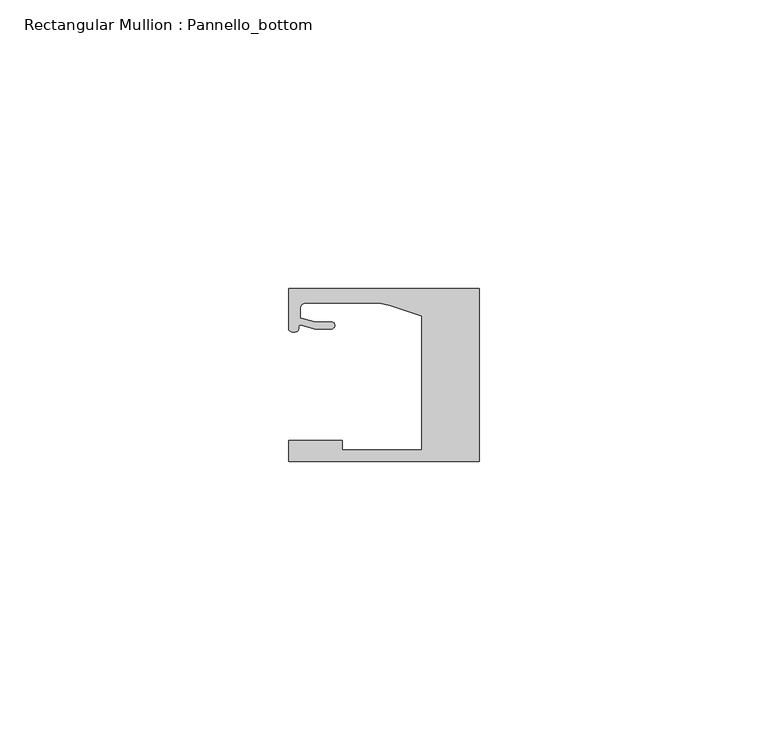
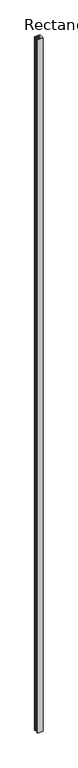
"""IFC4 building model written with IfcOpenShell, lengths in millimetres: member geometry, Rectangular Mullion : Pannello_bottom."""

import ifcopenshell
import ifcopenshell.guid

model = None  # the IFC model being written
_history = None  # IfcOwnerHistory: only IFC2X3 demands one
_inside = {}  # id of a spatial element -> (the spatial element, [elements in it])
_under = {}  # id of a project, library or spatial element -> (it, [spatial elements below it])
_declared = {}  # id of a project -> (the project, [libraries it declares])
_typed = {}  # id of a type object -> (the type object, [elements of that type])
_made_of = {}  # id of a material, layer set ... -> (it, [elements and type objects made of it])


def new_model(schema):
    """Start an empty IFC model of exactly this schema.

    Asked for "IFC4X3", IfcOpenShell would pick the latest addendum, in which some entities
    have other attributes; the version numbers below select the first issue.
    IFC2X3 requires an IfcOwnerHistory on every rooted entity: one is made here for all.
    """
    global model, _history
    if schema == "IFC4X3":
        model = ifcopenshell.file(schema_version=(4, 3, 0, 0))
    else:
        model = ifcopenshell.file(schema=schema)
    _inside.clear()
    _under.clear()
    _declared.clear()
    _typed.clear()
    _made_of.clear()
    _history = None
    if model.schema == "IFC2X3":
        org = make("IfcOrganization", Name="unknown")
        user = make(
            "IfcPersonAndOrganization",
            ThePerson=make("IfcPerson", FamilyName="unknown"),
            TheOrganization=org,
        )
        app = make(
            "IfcApplication",
            ApplicationDeveloper=org,
            Version="unknown",
            ApplicationFullName="unknown",
            ApplicationIdentifier="unknown",
        )
        _history = make(
            "IfcOwnerHistory",
            OwningUser=user,
            OwningApplication=app,
            ChangeAction="ADDED",
            CreationDate=0,
        )
    return model


def make(cls, **values):
    """One entity of the class cls with the attributes given. An attribute that is None is left unset."""
    return model.create_entity(
        cls, **{name: value for name, value in values.items() if value is not None}
    )


def rooted(cls, **values):
    """An entity with a GlobalId (a new one), such as an element, a storey or a relation."""
    return make(cls, GlobalId=ifcopenshell.guid.new(), OwnerHistory=_history, **values)


def si_unit(unit_type, name, prefix=None):
    """IfcSIUnit, for example si_unit("LENGTHUNIT", "METRE", prefix="MILLI")."""
    return make("IfcSIUnit", UnitType=unit_type, Prefix=prefix, Name=name)


def assignment(units):
    """IfcUnitAssignment: the units of a project."""
    return None if units is None else make("IfcUnitAssignment", Units=units)


def point(xyz):
    """IfcCartesianPoint."""
    return None if xyz is None else make("IfcCartesianPoint", Coordinates=xyz)


def direction(xyz):
    """IfcDirection."""
    return None if xyz is None else make("IfcDirection", DirectionRatios=xyz)


def frame(location, z_axis=None, x_axis=None):
    """IfcAxis2Placement3D, a coordinate frame: its origin and axes. An axis left out is left unset."""
    return make(
        "IfcAxis2Placement3D",
        Location=point(location),
        Axis=direction(z_axis),
        RefDirection=direction(x_axis),
    )


def origin():
    """The frame at (0, 0, 0) with its axes left unset."""
    return frame((0.0, 0.0, 0.0))


def place(relative_to, where):
    """IfcLocalPlacement: puts the frame where relative to a parent placement (None: the world)."""
    return make(
        "IfcLocalPlacement", PlacementRelTo=relative_to, RelativePlacement=where
    )


def context(
    kind, dimensions, precision=None, world=None, true_north=None, identifier=None
):
    """IfcGeometricRepresentationContext, for example the 3D "Model" context."""
    return make(
        "IfcGeometricRepresentationContext",
        ContextIdentifier=identifier,
        ContextType=kind,
        CoordinateSpaceDimension=dimensions,
        Precision=precision,
        WorldCoordinateSystem=world,
        TrueNorth=true_north,
    )


def project(units=None, contexts=None):
    """IfcProject with its units and contexts."""
    return rooted(
        "IfcProject",
        Name="project",
        RepresentationContexts=contexts,
        UnitsInContext=assignment(units),
    )


def spatial(cls, under=None, at=None, **own):
    """A site, building, storey or space (cls), placed at a placement, below another one or the project."""
    s = rooted(cls, ObjectPlacement=at, **own)
    if under is not None:
        _under.setdefault(under.id(), (under, []))[1].append(s)
    return s


def polyline(points):
    """IfcPolyline through the points."""
    return make("IfcPolyline", Points=[point(p) for p in points])


def circle_curve(where, radius):
    """IfcCircle in the frame where."""
    return make("IfcCircle", Position=where, Radius=radius)


def shape(context_of_items, identifier, shape_type, items):
    """IfcShapeRepresentation: the items that make up one representation, for example the "Body"."""
    return make(
        "IfcShapeRepresentation",
        ContextOfItems=context_of_items,
        RepresentationIdentifier=identifier,
        RepresentationType=shape_type,
        Items=items,
    )


def source(mapping_origin, context_of_items, identifier, shape_type, items):
    """IfcRepresentationMap: a shape defined once, which mapped items show again and again."""
    return make(
        "IfcRepresentationMap",
        MappingOrigin=mapping_origin,
        MappedRepresentation=shape(context_of_items, identifier, shape_type, items),
    )


def transform(
    local_origin,
    x_axis=None,
    y_axis=None,
    z_axis=None,
    scale=None,
    scale2=None,
    scale3=None,
    uniform=True,
):
    """IfcCartesianTransformationOperator3D, or its non-uniform kind. x_axis, y_axis, z_axis: its Axis1, 2, 3."""
    if uniform:
        return make(
            "IfcCartesianTransformationOperator3D",
            Axis1=direction(x_axis),
            Axis2=direction(y_axis),
            LocalOrigin=point(local_origin),
            Scale=scale,
            Axis3=direction(z_axis),
        )
    return make(
        "IfcCartesianTransformationOperator3DnonUniform",
        Axis1=direction(x_axis),
        Axis2=direction(y_axis),
        LocalOrigin=point(local_origin),
        Scale=scale,
        Axis3=direction(z_axis),
        Scale2=scale2,
        Scale3=scale3,
    )


def mapped(mapping_source, mapping_target):
    """IfcMappedItem: shows the shape of a source again, moved by a transform."""
    return make(
        "IfcMappedItem", MappingSource=mapping_source, MappingTarget=mapping_target
    )


def made_of(thing, what):
    """Note that an element or type object is made of a material, layer set ...; save() writes the relation."""
    if what is not None:
        _made_of.setdefault(what.id(), (what, []))[1].append(thing)
    return thing


def element(
    cls,
    number,
    at=None,
    inside=None,
    cuts=None,
    type_object=None,
    material=None,
    context=None,
    identifier="Body",
    shape_type=None,
    held_by="IfcProductDefinitionShape",
    body=None,
    shapes=None,
    **own,
):
    """One element of the class cls, such as IfcWall. Its Tag is "e" and its number.

    at: its placement. inside: the storey or other place that contains it. cuts: it is an
    opening in that element (IfcRelVoidsElement). A single representation is given by context,
    identifier, shape_type and body (its items); several are given by shapes. held_by: the class
    of the entity that holds the representations. save() writes the other relations.
    """
    e = rooted(cls, Tag="e%d" % number, ObjectPlacement=at, **own)
    if body is not None:
        shapes = [shape(context, identifier, shape_type, body)]
    if shapes is not None:
        e.Representation = make(held_by, Representations=shapes)
    if inside is not None:
        _inside.setdefault(inside.id(), (inside, []))[1].append(e)
    if cuts is not None:
        rooted(
            "IfcRelVoidsElement", RelatingBuildingElement=cuts, RelatedOpeningElement=e
        )
    if type_object is not None:
        _typed.setdefault(type_object.id(), (type_object, []))[1].append(e)
    return made_of(e, material)


def aggregate(whole, parts):
    """IfcRelAggregates: a whole, such as a stair, and the parts it consists of."""
    return rooted("IfcRelAggregates", RelatingObject=whole, RelatedObjects=parts)


def save(model, path):
    """Write the relations noted so far, then the file.

    IfcRelAggregates (storeys below a building ...), IfcRelContainedInSpatialStructure (elements
    in a storey), IfcRelDefinesByType, IfcRelAssociatesMaterial and IfcRelDeclares: one each for
    every whole, place, type object, material and project.
    """
    for whole, parts in _under.values():
        aggregate(whole, parts)
    for where, things in _inside.values():
        rooted(
            "IfcRelContainedInSpatialStructure",
            RelatedElements=things,
            RelatingStructure=where,
        )
    for kind, things in _typed.values():
        rooted("IfcRelDefinesByType", RelatedObjects=things, RelatingType=kind)
    for what, things in _made_of.values():
        rooted("IfcRelAssociatesMaterial", RelatedObjects=things, RelatingMaterial=what)
    for by, libraries in _declared.values():
        rooted("IfcRelDeclares", RelatingContext=by, RelatedDefinitions=libraries)
    model.write(path)


def plane_surface(at):
    """IfcPlane: the flat surface through the origin of the frame at, square to its z axis."""
    return make("IfcPlane", Position=at)


def cylinder_surface(at, radius):
    """IfcCylindricalSurface: all points at the distance radius from the z axis of the frame at."""
    return make("IfcCylindricalSurface", Position=at, Radius=radius)


def revolved_surface(curve, axis_point, axis_direction):
    """IfcSurfaceOfRevolution: the curve turned about the line through axis_point along axis_direction."""
    return make(
        "IfcSurfaceOfRevolution",
        SweptCurve=make("IfcArbitraryOpenProfileDef", ProfileType="CURVE", Curve=curve),
        AxisPosition=make("IfcAxis1Placement", Location=point(axis_point), Axis=direction(axis_direction)),
    )


def extruded_surface(curve, direction_of_extrusion, depth):
    """IfcSurfaceOfLinearExtrusion: the curve pushed along a direction by depth."""
    return make(
        "IfcSurfaceOfLinearExtrusion",
        SweptCurve=make("IfcArbitraryOpenProfileDef", ProfileType="CURVE", Curve=curve),
        ExtrudedDirection=direction(direction_of_extrusion),
        Depth=depth,
    )


def spline_curve(degree, points, multiplicities, knots, weights=None):
    """IfcBSplineCurveWithKnots; with weights, IfcRationalBSplineCurveWithKnots."""
    own = dict(
        Degree=degree,
        ControlPointsList=[point(p) for p in points],
        CurveForm="UNSPECIFIED",
        ClosedCurve=False,
        SelfIntersect=False,
        KnotMultiplicities=multiplicities,
        Knots=knots,
        KnotSpec="UNSPECIFIED",
    )
    if weights is None:
        return make("IfcBSplineCurveWithKnots", **own)
    return make("IfcRationalBSplineCurveWithKnots", WeightsData=weights, **own)


def advanced_brep(points, edges, surfaces, faces):
    """IfcAdvancedBrep: a solid bounded by faces that lie on surfaces and meet in shared edges.

    An edge is (start, end): straight between two places in points (the first is 0);
    or (start, end, curve); or (start, end, curve, False) where it runs against its curve.
    A face is (place in surfaces, loops), or (place, loops, False) where it looks against
    its surface's normal. A loop lists edges by number (the first is 1), with a minus sign
    where the edge is run from its end to its start. The first loop is the outer one.
    """
    corners = [point(p) for p in points]
    vertices = [make("IfcVertexPoint", VertexGeometry=c) for c in corners]
    made = []
    for start, end, *more in edges:
        made.append(
            make(
                "IfcEdgeCurve",
                EdgeStart=vertices[start],
                EdgeEnd=vertices[end],
                EdgeGeometry=more[0] if more else make("IfcPolyline", Points=[corners[start], corners[end]]),
                SameSense=more[1] if len(more) > 1 else True,
            )
        )
    hull = []
    for where, loops, *sense in faces:
        bounds = []
        for j, loop in enumerate(loops):
            ring = [make("IfcOrientedEdge", EdgeElement=made[abs(k) - 1], Orientation=k > 0) for k in loop]
            bounds.append(
                make(
                    "IfcFaceOuterBound" if j == 0 else "IfcFaceBound",
                    Bound=make("IfcEdgeLoop", EdgeList=ring),
                    Orientation=True,
                )
            )
        hull.append(make("IfcAdvancedFace", Bounds=bounds, FaceSurface=surfaces[where], SameSense=sense[0] if sense else True))
    return make("IfcAdvancedBrep", Outer=make("IfcClosedShell", CfsFaces=hull))


def rectangular_mullion_pannello_bottom_0b2f488d(model_context):
    return source(origin(), model_context, "Body", "AdvancedBrep", [
        advanced_brep(
        [(-33.0, -15.0, 0.0), (0.0, -15.0, 0.0), (0.0, 15.0, 0.0), (-33.0000135, 15.0, 0.0), (-33.0000135, 8.0000472, 0.0), (-30.9223017, 8.6490241, 0.0), (-28.4999305, 7.9999523, 0.0), (-25.59998, 7.9999523, 0.0), (-25.59998, 9.1999523, 0.0), (-28.3419477, 9.1999523, 0.0), (-31.0, 9.9121746, 0.0), (-31.0, 11.4999419, 0.0), (-30.0000002, 12.4999419, 0.0), (-18.5493024, 12.4999438, 0.0), (-15.4591336, 12.0105099, 0.0), (-9.9999723, 10.2367227, 0.0), (-9.9999723, -13.0000004, 0.0), (-23.700041, -13.0000004, 0.0), (-23.700041, -11.3000004, 0.0), (-33.0, -11.3000004, 0.0), (-33.0, -15.0, -4398.2697983), (-33.0, -11.3000004, -4398.2697983), (-23.700041, -11.3000004, -4398.2697983), (-23.700041, -13.0000004, -4398.2697983), (-9.9999723, -13.0000004, -4398.2697983), (-9.9999723, 10.2367227, -4398.2697983), (-15.4591336, 12.0105099, -4398.2697983), (-18.5493024, 12.4999438, -4398.2697983), (-30.0000002, 12.4999419, -4398.2697983), (-31.0, 11.4999419, -4398.2697983), (-31.0, 9.9121746, -4398.2697983), (-28.3419477, 9.1999523, -4398.2697983), (-25.59998, 9.1999523, -4398.2697983), (-25.59998, 7.9999523, -4398.2697983), (-28.4999305, 7.9999523, -4398.2697983), (-30.9223017, 8.6490241, -4398.2697983), (-33.0000135, 8.0000472, -4398.2697983), (-33.0000135, 15.0, -4398.2697983), (0.0, 15.0, -4398.2697983), (0.0, -15.0, -4398.2697983)],
        [
            (0, 1),
            (1, 2),
            (2, 3),
            (3, 4),
            (4, 5, spline_curve(3, [(-33.0000135, 8.0000472, 0.0), (-33.0000135, 7.457047519, 0.0), (-32.262327879, 7.456527435, 0.0), (-31.357433266, 7.563996614, 0.0), (-31.305645054, 7.690065204, 0.0), (-31.298563602, 8.366228555, 0.0), (-31.312054066, 8.717747958, 0.0), (-30.9223017, 8.6490241, 0.0)], [4, 2, 2, 4], [0.0, 0.0027053965905959043, 0.0058611956533709, 0.007702013405570312])),
            (5, 6),
            (6, 7),
            (7, 8, circle_curve(frame((-25.59998, 8.5999523, 0.0), z_axis=(0.0, 0.0, 1.0), x_axis=(0.0, 1.0, 0.0)), 0.6)),
            (8, 9),
            (9, 10),
            (10, 11),
            (11, 12, circle_curve(frame((-30.0, 11.4999419, 0.0), z_axis=(0.0, 0.0, -1.0), x_axis=(0.0, 1.0, 0.0)), 1.0)),
            (12, 13),
            (13, 14, circle_curve(frame((-18.5493007, 2.4999438, 0.0), z_axis=(0.0, 0.0, -1.0), x_axis=(0.0, 1.0, 0.0)), 10.0)),
            (14, 15),
            (15, 16),
            (16, 17),
            (17, 18),
            (18, 19),
            (19, 0),
            (20, 21),
            (21, 22),
            (22, 23),
            (23, 24),
            (24, 25),
            (25, 26),
            (26, 27, circle_curve(frame((-18.5493007, 2.4999438, -4398.2697983), z_axis=(0.0, 0.0, 1.0), x_axis=(0.0, 1.0, 0.0)), 10.0)),
            (27, 28),
            (28, 29, circle_curve(frame((-30.0, 11.4999419, -4398.2697983), z_axis=(0.0, 0.0, 1.0), x_axis=(0.0, 1.0, 0.0)), 1.0)),
            (29, 30),
            (30, 31),
            (31, 32),
            (32, 33, circle_curve(frame((-25.59998, 8.5999523, -4398.2697983), z_axis=(0.0, 0.0, -1.0), x_axis=(0.0, 1.0, 0.0)), 0.6)),
            (33, 34),
            (34, 35),
            (35, 36, spline_curve(3, [(-30.9223017, 8.6490241, -4398.2697983), (-31.312054066, 8.717747958, -4398.2697983), (-31.298563602, 8.366228555, -4398.2697983), (-31.305645054, 7.690065204, -4398.2697983), (-31.357433266, 7.563996614, -4398.2697983), (-32.262327879, 7.456527435, -4398.2697983), (-33.0000135, 7.457047519, -4398.2697983), (-33.0000135, 8.0000472, -4398.2697983)], [4, 2, 2, 4], [0.0, 0.001840817752199412, 0.004996616814974408, 0.007702013405570312])),
            (36, 37),
            (37, 38),
            (38, 39),
            (39, 20),
            (0, 20),
            (39, 1),
            (38, 2),
            (37, 3),
            (36, 4),
            (35, 5),
            (34, 6),
            (33, 7),
            (32, 8),
            (31, 9),
            (30, 10),
            (29, 11),
            (28, 12),
            (27, 13),
            (26, 14),
            (25, 15),
            (24, 16),
            (23, 17),
            (22, 18),
            (21, 19),
        ],
        [
            plane_surface(frame((0.0, -36.2491502, 0.0), z_axis=(0.0, 0.0, 1.0), x_axis=(-1.0, 0.0, 0.0))),
            plane_surface(frame((0.0, -36.2491502, -4398.2697983), z_axis=(0.0, 0.0, -1.0), x_axis=(-1.0, 0.0, 0.0))),
            plane_surface(frame((-33.0, -15.0, 0.0), z_axis=(0.0, -1.0, 0.0), x_axis=(0.0, 0.0, -1.0))),
            plane_surface(frame((0.0, -15.0, 0.0), z_axis=(1.0, 0.0, 0.0), x_axis=(0.0, 0.0, -1.0))),
            plane_surface(frame((0.0, 15.0, 0.0), z_axis=(0.0, 1.0, 0.0), x_axis=(0.0, 0.0, -1.0))),
            plane_surface(frame((-33.0000135, 15.0, 0.0), z_axis=(-1.0, 0.0, 0.0), x_axis=(0.0, 0.0, -1.0))),
            extruded_surface(spline_curve(3, [(-33.0000135, 8.0000472, -4398.2697983), (-33.0000135, 7.457047519, -4398.2697983), (-32.262327879, 7.456527435, -4398.2697983), (-31.357433266, 7.563996614, -4398.2697983), (-31.305645054, 7.690065204, -4398.2697983), (-31.298563602, 8.366228555, -4398.2697983), (-31.312054066, 8.717747958, -4398.2697983), (-30.9223017, 8.6490241, -4398.2697983)], [4, 2, 2, 4], [0.0, 0.0027053965905959043, 0.0058611956533709, 0.007702013405570312]), (0.0, 0.0, 4398.2697983), 4398.2697983),
            plane_surface(frame((-30.9223017, 8.6490241, 0.0), z_axis=(-0.25881883200192934, -0.9659258833891746, 0.0), x_axis=(0.0, 0.0, -1.0))),
            plane_surface(frame((-28.4999305, 7.9999523, 0.0), z_axis=(0.0, -1.0, 0.0), x_axis=(0.0, 0.0, -1.0))),
            cylinder_surface(frame((-25.59998, 8.5999523, 0.0), z_axis=(0.0, 0.0, 1.0), x_axis=(0.0, 1.0, 0.0)), 0.6),
            plane_surface(frame((-25.59998, 9.1999523, 0.0), z_axis=(0.0, 1.0, 0.0), x_axis=(0.0, 0.0, -1.0))),
            plane_surface(frame((-28.3419477, 9.1999523, 0.0), z_axis=(0.25881883204288636, 0.9659258833782002, 0.0), x_axis=(0.0, 0.0, -1.0))),
            plane_surface(frame((-31.0, 9.9121746, 0.0), z_axis=(1.0, 0.0, 0.0), x_axis=(0.0, 0.0, -1.0))),
            revolved_surface(polyline([(-30.0, 12.4999419, -4398.2697983), (-30.0, 12.4999419, 0.0)]), (-30.0, 11.4999419, 0.0), (0.0, 0.0, -1.0)),
            plane_surface(frame((-30.0000002, 12.4999419, 0.0), z_axis=(1.6923026533778639e-07, -0.9999999999999858, 0.0), x_axis=(0.0, 0.0, -1.0))),
            revolved_surface(polyline([(-18.5493007, 12.4999438, -4398.2697983), (-18.5493007, 12.4999438, 0.0)]), (-18.5493007, 2.4999438, 0.0), (0.0, 0.0, -1.0)),
            plane_surface(frame((-15.4591336, 12.0105099, 0.0), z_axis=(-0.30901670911956314, -0.9510566089801992, 0.0), x_axis=(0.0, 0.0, -1.0))),
            plane_surface(frame((-9.9999723, 10.2367227, 0.0), z_axis=(-1.0, 0.0, 0.0), x_axis=(0.0, 0.0, -1.0))),
            plane_surface(frame((-9.9999723, -13.0000004, 0.0), z_axis=(0.0, 1.0, 0.0), x_axis=(0.0, 0.0, -1.0))),
            plane_surface(frame((-23.700041, -13.0000004, 0.0), z_axis=(1.0, 0.0, 0.0), x_axis=(0.0, 0.0, -1.0))),
            plane_surface(frame((-23.700041, -11.3000004, 0.0), z_axis=(0.0, 1.0, 0.0), x_axis=(0.0, 0.0, -1.0))),
            plane_surface(frame((-33.0, -11.3000004, 0.0), z_axis=(-1.0, 0.0, 0.0), x_axis=(0.0, 0.0, -1.0))),
        ],
        [
            (0, [[1, 2, 3, 4, 5, 6, 7, 8, 9, 10, 11, 12, 13, 14, 15, 16, 17, 18, 19, 20]]),
            (1, [[21, 22, 23, 24, 25, 26, 27, 28, 29, 30, 31, 32, 33, 34, 35, 36, 37, 38, 39, 40]]),
            (2, [[-1, 41, -40, 42]]),
            (3, [[-2, -42, -39, 43]]),
            (4, [[-3, -43, -38, 44]]),
            (5, [[-4, -44, -37, 45]]),
            (6, [[-5, -45, -36, 46]]),
            (7, [[-6, -46, -35, 47]]),
            (8, [[-7, -47, -34, 48]]),
            (9, [[-8, -48, -33, 49]]),
            (10, [[-9, -49, -32, 50]]),
            (11, [[-10, -50, -31, 51]]),
            (12, [[-11, -51, -30, 52]]),
            (13, [[-12, -52, -29, 53]]),
            (14, [[-13, -53, -28, 54]]),
            (15, [[-14, -54, -27, 55]]),
            (16, [[-15, -55, -26, 56]]),
            (17, [[-16, -56, -25, 57]]),
            (18, [[-17, -57, -24, 58]]),
            (19, [[-18, -58, -23, 59]]),
            (20, [[-19, -59, -22, 60]]),
            (21, [[-20, -60, -21, -41]]),
        ],
    ),
    ])


if __name__ == "__main__":
    model = new_model("IFC4")
    model_context = context("Model", 3, world=origin())
    ifc_project = project(units=[si_unit("LENGTHUNIT", "METRE", prefix="MILLI")], contexts=[model_context])
    site = spatial("IfcSite", under=ifc_project)
    building = spatial("IfcBuilding", under=site)
    placement = place(None, origin())
    rectangular_mullion_pannello_bottom_shape = rectangular_mullion_pannello_bottom_0b2f488d(model_context)
    element("IfcMember", 1, ObjectType="Rectangular Mullion : Pannello_bottom", at=placement, inside=building, context=model_context, shape_type="MappedRepresentation", body=[
        mapped(rectangular_mullion_pannello_bottom_shape, transform((0.0, 0.0, 0.0), x_axis=(1.0, 0.0, 0.0), y_axis=(0.0, 1.0, 0.0), z_axis=(0.0, 0.0, 1.0))),
    ])
    save(model, "model.ifc")

# Revit data of these elements
# Type "Rectangular Mullion : Pannello_bottom"
#   built-in parameter 1007322 = 0.0984252 (stored number, unit not read)
#   built-in parameter 1007321 = 0.0328083 (stored number, unit not read)
#   built-in parameter 1007320 = 0 (stored number, unit not read)
